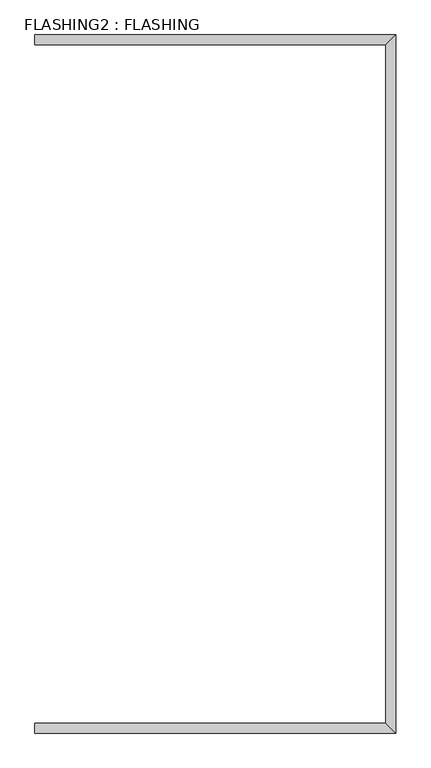
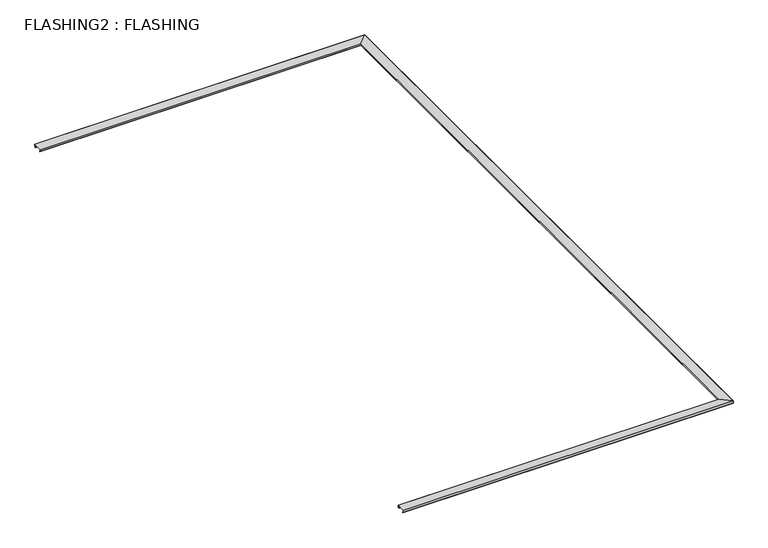
"""IFC4 building model written with IfcOpenShell, lengths in millimetres: proxy geometry, FLASHING2 : FLASHING."""

import ifcopenshell
import ifcopenshell.guid

model = None  # the IFC model being written
_history = None  # IfcOwnerHistory: only IFC2X3 demands one
_inside = {}  # id of a spatial element -> (the spatial element, [elements in it])
_under = {}  # id of a project, library or spatial element -> (it, [spatial elements below it])
_declared = {}  # id of a project -> (the project, [libraries it declares])
_typed = {}  # id of a type object -> (the type object, [elements of that type])
_made_of = {}  # id of a material, layer set ... -> (it, [elements and type objects made of it])


def new_model(schema):
    """Start an empty IFC model of exactly this schema.

    Asked for "IFC4X3", IfcOpenShell would pick the latest addendum, in which some entities
    have other attributes; the version numbers below select the first issue.
    IFC2X3 requires an IfcOwnerHistory on every rooted entity: one is made here for all.
    """
    global model, _history
    if schema == "IFC4X3":
        model = ifcopenshell.file(schema_version=(4, 3, 0, 0))
    else:
        model = ifcopenshell.file(schema=schema)
    _inside.clear()
    _under.clear()
    _declared.clear()
    _typed.clear()
    _made_of.clear()
    _history = None
    if model.schema == "IFC2X3":
        org = make("IfcOrganization", Name="unknown")
        user = make(
            "IfcPersonAndOrganization",
            ThePerson=make("IfcPerson", FamilyName="unknown"),
            TheOrganization=org,
        )
        app = make(
            "IfcApplication",
            ApplicationDeveloper=org,
            Version="unknown",
            ApplicationFullName="unknown",
            ApplicationIdentifier="unknown",
        )
        _history = make(
            "IfcOwnerHistory",
            OwningUser=user,
            OwningApplication=app,
            ChangeAction="ADDED",
            CreationDate=0,
        )
    return model


def make(cls, **values):
    """One entity of the class cls with the attributes given. An attribute that is None is left unset."""
    return model.create_entity(
        cls, **{name: value for name, value in values.items() if value is not None}
    )


def rooted(cls, **values):
    """An entity with a GlobalId (a new one), such as an element, a storey or a relation."""
    return make(cls, GlobalId=ifcopenshell.guid.new(), OwnerHistory=_history, **values)


def si_unit(unit_type, name, prefix=None):
    """IfcSIUnit, for example si_unit("LENGTHUNIT", "METRE", prefix="MILLI")."""
    return make("IfcSIUnit", UnitType=unit_type, Prefix=prefix, Name=name)


def assignment(units):
    """IfcUnitAssignment: the units of a project."""
    return None if units is None else make("IfcUnitAssignment", Units=units)


def point(xyz):
    """IfcCartesianPoint."""
    return None if xyz is None else make("IfcCartesianPoint", Coordinates=xyz)


def direction(xyz):
    """IfcDirection."""
    return None if xyz is None else make("IfcDirection", DirectionRatios=xyz)


def frame(location, z_axis=None, x_axis=None):
    """IfcAxis2Placement3D, a coordinate frame: its origin and axes. An axis left out is left unset."""
    return make(
        "IfcAxis2Placement3D",
        Location=point(location),
        Axis=direction(z_axis),
        RefDirection=direction(x_axis),
    )


def origin():
    """The frame at (0, 0, 0) with its axes left unset."""
    return frame((0.0, 0.0, 0.0))


def place(relative_to, where):
    """IfcLocalPlacement: puts the frame where relative to a parent placement (None: the world)."""
    return make(
        "IfcLocalPlacement", PlacementRelTo=relative_to, RelativePlacement=where
    )


def context(
    kind, dimensions, precision=None, world=None, true_north=None, identifier=None
):
    """IfcGeometricRepresentationContext, for example the 3D "Model" context."""
    return make(
        "IfcGeometricRepresentationContext",
        ContextIdentifier=identifier,
        ContextType=kind,
        CoordinateSpaceDimension=dimensions,
        Precision=precision,
        WorldCoordinateSystem=world,
        TrueNorth=true_north,
    )


def project(units=None, contexts=None):
    """IfcProject with its units and contexts."""
    return rooted(
        "IfcProject",
        Name="project",
        RepresentationContexts=contexts,
        UnitsInContext=assignment(units),
    )


def spatial(cls, under=None, at=None, **own):
    """A site, building, storey or space (cls), placed at a placement, below another one or the project."""
    s = rooted(cls, ObjectPlacement=at, **own)
    if under is not None:
        _under.setdefault(under.id(), (under, []))[1].append(s)
    return s


def faces_of(points, faces, orient=None, outer=None):
    """IfcFace entities. A face is a list of loops; a loop is a list of indices into points, from 0.

    orient and outer hold one flag for each loop. By default every Orientation is true, the
    first loop of a face is its IfcFaceOuterBound and the others are IfcFaceBound.
    """
    made = []
    for i, loops in enumerate(faces):
        bounds = []
        for j, loop in enumerate(loops):
            is_outer = j == 0 if outer is None else outer[i][j]
            bounds.append(
                make(
                    "IfcFaceOuterBound" if is_outer else "IfcFaceBound",
                    Bound=make("IfcPolyLoop", Polygon=[points[k] for k in loop]),
                    Orientation=True if orient is None else orient[i][j],
                )
            )
        made.append(make("IfcFace", Bounds=bounds))
    return made


def faceted_brep(points, faces, orient=None, outer=None, voids=None):
    """IfcFacetedBrep: a solid bounded by flat faces; with voids (closed shells), ...WithVoids."""
    shared = [point(p) for p in points]
    hull = make("IfcClosedShell", CfsFaces=faces_of(shared, faces, orient, outer))
    if voids is None:
        return make("IfcFacetedBrep", Outer=hull)
    return make(
        "IfcFacetedBrepWithVoids",
        Outer=hull,
        Voids=[
            make(cls, CfsFaces=faces_of(shared, fs, o, b)) for cls, fs, o, b in voids
        ],
    )


def shape(context_of_items, identifier, shape_type, items):
    """IfcShapeRepresentation: the items that make up one representation, for example the "Body"."""
    return make(
        "IfcShapeRepresentation",
        ContextOfItems=context_of_items,
        RepresentationIdentifier=identifier,
        RepresentationType=shape_type,
        Items=items,
    )


def source(mapping_origin, context_of_items, identifier, shape_type, items):
    """IfcRepresentationMap: a shape defined once, which mapped items show again and again."""
    return make(
        "IfcRepresentationMap",
        MappingOrigin=mapping_origin,
        MappedRepresentation=shape(context_of_items, identifier, shape_type, items),
    )


def transform(
    local_origin,
    x_axis=None,
    y_axis=None,
    z_axis=None,
    scale=None,
    scale2=None,
    scale3=None,
    uniform=True,
):
    """IfcCartesianTransformationOperator3D, or its non-uniform kind. x_axis, y_axis, z_axis: its Axis1, 2, 3."""
    if uniform:
        return make(
            "IfcCartesianTransformationOperator3D",
            Axis1=direction(x_axis),
            Axis2=direction(y_axis),
            LocalOrigin=point(local_origin),
            Scale=scale,
            Axis3=direction(z_axis),
        )
    return make(
        "IfcCartesianTransformationOperator3DnonUniform",
        Axis1=direction(x_axis),
        Axis2=direction(y_axis),
        LocalOrigin=point(local_origin),
        Scale=scale,
        Axis3=direction(z_axis),
        Scale2=scale2,
        Scale3=scale3,
    )


def mapped(mapping_source, mapping_target):
    """IfcMappedItem: shows the shape of a source again, moved by a transform."""
    return make(
        "IfcMappedItem", MappingSource=mapping_source, MappingTarget=mapping_target
    )


def made_of(thing, what):
    """Note that an element or type object is made of a material, layer set ...; save() writes the relation."""
    if what is not None:
        _made_of.setdefault(what.id(), (what, []))[1].append(thing)
    return thing


def element(
    cls,
    number,
    at=None,
    inside=None,
    cuts=None,
    type_object=None,
    material=None,
    context=None,
    identifier="Body",
    shape_type=None,
    held_by="IfcProductDefinitionShape",
    body=None,
    shapes=None,
    **own,
):
    """One element of the class cls, such as IfcWall. Its Tag is "e" and its number.

    at: its placement. inside: the storey or other place that contains it. cuts: it is an
    opening in that element (IfcRelVoidsElement). A single representation is given by context,
    identifier, shape_type and body (its items); several are given by shapes. held_by: the class
    of the entity that holds the representations. save() writes the other relations.
    """
    e = rooted(cls, Tag="e%d" % number, ObjectPlacement=at, **own)
    if body is not None:
        shapes = [shape(context, identifier, shape_type, body)]
    if shapes is not None:
        e.Representation = make(held_by, Representations=shapes)
    if inside is not None:
        _inside.setdefault(inside.id(), (inside, []))[1].append(e)
    if cuts is not None:
        rooted(
            "IfcRelVoidsElement", RelatingBuildingElement=cuts, RelatedOpeningElement=e
        )
    if type_object is not None:
        _typed.setdefault(type_object.id(), (type_object, []))[1].append(e)
    return made_of(e, material)


def aggregate(whole, parts):
    """IfcRelAggregates: a whole, such as a stair, and the parts it consists of."""
    return rooted("IfcRelAggregates", RelatingObject=whole, RelatedObjects=parts)


def save(model, path):
    """Write the relations noted so far, then the file.

    IfcRelAggregates (storeys below a building ...), IfcRelContainedInSpatialStructure (elements
    in a storey), IfcRelDefinesByType, IfcRelAssociatesMaterial and IfcRelDeclares: one each for
    every whole, place, type object, material and project.
    """
    for whole, parts in _under.values():
        aggregate(whole, parts)
    for where, things in _inside.values():
        rooted(
            "IfcRelContainedInSpatialStructure",
            RelatedElements=things,
            RelatingStructure=where,
        )
    for kind, things in _typed.values():
        rooted("IfcRelDefinesByType", RelatedObjects=things, RelatingType=kind)
    for what, things in _made_of.values():
        rooted("IfcRelAssociatesMaterial", RelatedObjects=things, RelatingMaterial=what)
    for by, libraries in _declared.values():
        rooted("IfcRelDeclares", RelatingContext=by, RelatedDefinitions=libraries)
    model.write(path)


def flashing2_flashing_8f2ab91a(model_context):
    return source(origin(), model_context, "Body", "Brep", [
        faceted_brep([(50865.0, 39914.5208589, 7739.9720055), (50865.0, 39914.5208589, 7724.9720055), (50865.0, 20084.5208589, 7724.9720055), (50865.0, 20084.5208589, 7739.9720055), (50866.0, 39915.5208589, 7750.9720055), (50866.0, 39915.5208589, 7739.9720055), (50866.0, 20083.5208589, 7739.9720055), (50866.0, 20083.5208589, 7750.9720055), (50894.0, 39943.5208589, 7819.1280996), (50894.0, 39943.5208589, 7750.9720055), (50894.0, 20055.5208589, 7750.9720055), (50894.0, 20055.5208589, 7819.1280996), (50611.0, 39660.5208589, 7808.0300604), (50611.0, 20338.5208589, 7808.0300604), (50611.0, 39660.5208589, 7750.9720055), (50611.0, 20338.5208589, 7750.9720055), (50639.0, 39688.5208589, 7739.9720055), (50639.0, 39688.5208589, 7750.9720055), (50639.0, 20310.5208589, 7750.9720055), (50639.0, 20310.5208589, 7739.9720055), (50640.0, 39689.5208589, 7724.9720055), (50640.0, 39689.5208589, 7739.9720055), (50640.0, 20309.5208589, 7739.9720055), (50640.0, 20309.5208589, 7724.9720055), (50638.0, 39687.5208589, 7749.9720055), (50638.0, 39687.5208589, 7724.9720055), (50638.0, 20311.5208589, 7724.9720055), (50638.0, 20311.5208589, 7749.9720055), (50610.0, 39659.5208589, 7808.9916134), (50610.0, 39659.5208589, 7749.9720055), (50610.0, 20339.5208589, 7749.9720055), (50610.0, 20339.5208589, 7808.9916134), (50895.0, 39944.5208589, 7820.168084), (50895.0, 20054.5208589, 7820.168084), (50895.0, 39944.5208589, 7749.9720055), (50895.0, 20054.5208589, 7749.9720055), (50867.0, 39916.5208589, 7724.9720055), (50867.0, 39916.5208589, 7749.9720055), (50867.0, 20082.5208589, 7749.9720055), (50867.0, 20082.5208589, 7724.9720055), (40619.0, 20084.5208589, 7724.9720055), (40619.0, 20084.5208589, 7739.9720055), (40619.0, 20083.5208589, 7739.9720055), (40619.0, 20083.5208589, 7750.9720055), (40619.0, 20055.5208589, 7750.9720055), (40619.0, 20055.5208589, 7819.1280996), (40619.0, 20338.5208589, 7808.0300604), (40619.0, 20338.5208589, 7750.9720055), (40619.0, 20310.5208589, 7750.9720055), (40619.0, 20310.5208589, 7739.9720055), (40619.0, 20309.5208589, 7739.9720055), (40619.0, 20309.5208589, 7724.9720055), (40619.0, 20311.5208589, 7724.9720055), (40619.0, 20311.5208589, 7749.9720055), (40619.0, 20339.5208589, 7749.9720055), (40619.0, 20339.5208589, 7808.9916134), (40619.0, 20054.5208589, 7820.168084), (40619.0, 20054.5208589, 7749.9720055), (40619.0, 20082.5208589, 7749.9720055), (40619.0, 20082.5208589, 7724.9720055), (40619.0, 39914.5208589, 7739.9720055), (40619.0, 39914.5208589, 7724.9720055), (40619.0, 39915.5208589, 7739.9720055), (40619.0, 39915.5208589, 7750.9720055), (40619.0, 39943.5208589, 7750.9720055), (40619.0, 39943.5208589, 7819.1280996), (40619.0, 39660.5208589, 7808.0300604), (40619.0, 39660.5208589, 7750.9720055), (40619.0, 39688.5208589, 7750.9720055), (40619.0, 39688.5208589, 7739.9720055), (40619.0, 39689.5208589, 7739.9720055), (40619.0, 39689.5208589, 7724.9720055), (40619.0, 39687.5208589, 7724.9720055), (40619.0, 39687.5208589, 7749.9720055), (40619.0, 39659.5208589, 7749.9720055), (40619.0, 39659.5208589, 7808.9916134), (40619.0, 39944.5208589, 7820.168084), (40619.0, 39944.5208589, 7749.9720055), (40619.0, 39916.5208589, 7749.9720055), (40619.0, 39916.5208589, 7724.9720055)], [[[0, 1, 2, 3]], [[4, 5, 6, 7]], [[8, 9, 10, 11]], [[12, 8, 11, 13]], [[14, 12, 13, 15]], [[16, 17, 18, 19]], [[20, 21, 22, 23]], [[24, 25, 26, 27]], [[28, 29, 30, 31]], [[32, 28, 31, 33]], [[34, 32, 33, 35]], [[36, 37, 38, 39]], [[3, 2, 40, 41]], [[7, 6, 42, 43]], [[11, 10, 44, 45]], [[13, 11, 45, 46]], [[15, 13, 46, 47]], [[19, 18, 48, 49]], [[23, 22, 50, 51]], [[27, 26, 52, 53]], [[31, 30, 54, 55]], [[33, 31, 55, 56]], [[35, 33, 56, 57]], [[39, 38, 58, 59]], [[60, 61, 1, 0]], [[62, 60, 0, 3, 41, 42, 6, 5]], [[63, 62, 5, 4]], [[64, 63, 4, 7, 43, 44, 10, 9]], [[65, 64, 9, 8]], [[66, 65, 8, 12]], [[67, 66, 12, 14]], [[68, 67, 14, 15, 47, 48, 18, 17]], [[69, 68, 17, 16]], [[70, 69, 16, 19, 49, 50, 22, 21]], [[71, 70, 21, 20]], [[72, 71, 20, 23, 51, 52, 26, 25]], [[73, 72, 25, 24]], [[74, 73, 24, 27, 53, 54, 30, 29]], [[75, 74, 29, 28]], [[76, 75, 28, 32]], [[77, 76, 32, 34]], [[78, 77, 34, 35, 57, 58, 38, 37]], [[79, 78, 37, 36]], [[61, 79, 36, 39, 59, 40, 2, 1]], [[61, 60, 62, 63, 64, 65, 66, 67, 68, 69, 70, 71, 72, 73, 74, 75, 76, 77, 78, 79]], [[40, 59, 58, 57, 56, 55, 54, 53, 52, 51, 50, 49, 48, 47, 46, 45, 44, 43, 42, 41]]]),
    ])


if __name__ == "__main__":
    model = new_model("IFC4")
    model_context = context("Model", 3, world=origin())
    ifc_project = project(units=[si_unit("LENGTHUNIT", "METRE", prefix="MILLI")], contexts=[model_context])
    site = spatial("IfcSite", under=ifc_project)
    building = spatial("IfcBuilding", under=site)
    placement = place(None, origin())
    flashing2_flashing_shape = flashing2_flashing_8f2ab91a(model_context)
    element("IfcBuildingElementProxy", 1, Name="FLASHING2 : FLASHING", ObjectType="FLASHING2 : FLASHING", at=placement, inside=building, context=model_context, shape_type="MappedRepresentation", body=[
        mapped(flashing2_flashing_shape, transform((0.0, 0.0, 0.0), x_axis=(1.0, 0.0, 0.0), y_axis=(0.0, 1.0, 0.0), z_axis=(0.0, 0.0, 1.0))),
    ])
    save(model, "model.ifc")
